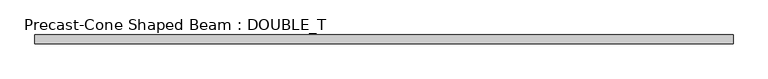
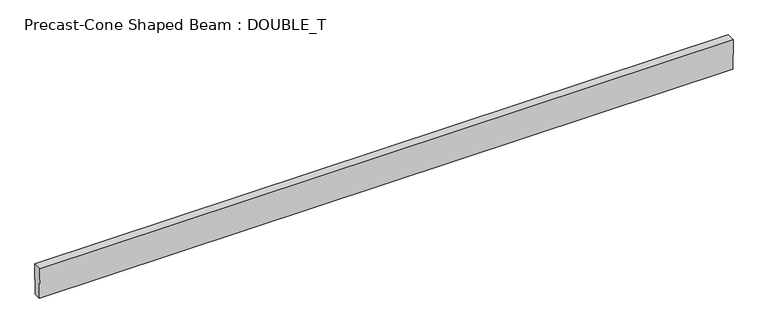
"""IFC4 building model written with IfcOpenShell, lengths in millimetres: beam geometry, Precast-Cone Shaped Beam : DOUBLE_T."""

from ifc_helpers import new_model, si_unit, frame, origin, place, context, project, spatial, polyline, outline, extrude, source, transform, mapped, element, save


def precast_cone_shaped_beam_double_t_a1b90a55(model_context):
    return source(origin(), model_context, "Body", "SweptSolid", [
        extrude(outline(polyline([(-50.8, -228.6), (-63.5, 228.6), (63.5, 228.6), (50.8, -228.6), (-50.8, -228.6)])), frame((-4891.88125, 0.0, 0.0), z_axis=(1.0, 0.0, 0.0), x_axis=(0.0, 1.0, 0.0)), (0.0, 0.0, 1.0), 10083.8),
    ])


if __name__ == "__main__":
    model = new_model("IFC4")
    model_context = context("Model", 3, world=origin())
    ifc_project = project(units=[si_unit("LENGTHUNIT", "METRE", prefix="MILLI")], contexts=[model_context])
    site = spatial("IfcSite", under=ifc_project)
    building = spatial("IfcBuilding", under=site)
    placement = place(None, origin())
    precast_cone_shaped_beam_double_t_shape = precast_cone_shaped_beam_double_t_a1b90a55(model_context)
    element("IfcBeam", 1, ObjectType="Precast-Cone Shaped Beam : DOUBLE_T", at=placement, inside=building, context=model_context, shape_type="MappedRepresentation", body=[
        mapped(precast_cone_shaped_beam_double_t_shape, transform((0.0, 0.0, 0.0), x_axis=(1.0, 0.0, 0.0), y_axis=(0.0, 1.0, 0.0), z_axis=(0.0, 0.0, 1.0))),
    ])
    save(model, "model.ifc")

# Revit data of these elements
# Type "Precast-Cone Shaped Beam : DOUBLE_T"
#   Top Width = 0' - 5"
#   Tie Rod Weight [instance default] = 30
#   Tie Rod W [instance default] = 0.0660938 kip
#   Single Rebar Weight [instance default] = 50
#   Single Rebar W [instance default] = 0.110156 kip
#   Rebar Grids Weight [instance default] = 100
#   Rebar Grids W [instance default] = 0.220313 kip
#   Depth = 1' - 6"
#   Bottom Width = 0' - 4"
#   Length [instance default] = 5' - 0"
#   Structural Material [instance default] = Concrete, Precast
#   Assembly Code = ""
# Element 1 (IfcBeam, "Precast-Cone Shaped Beam : DOUBLE_T")
#   Length = 33' - 1 3/16"
#   Structural Material = Concrete - Precast Concrete - Normal Weight Concrete - 5 ksi
#   Materials on its faces: "Concrete - Precast Concrete - Normal Weight Concrete - 5 ksi"
# Materials
#   "Concrete, Precast": class "Concrete", colour RGB 198 187 187, transparency 0, Description = "Precast concrete", Cost = 0
#   "Concrete - Precast Concrete - Normal Weight Concrete - 5 ksi": class "Concrete", colour RGB 198 187 187, transparency 0, Cost = 0
